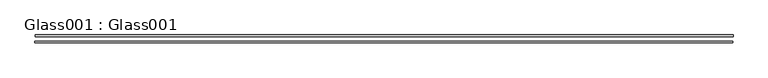
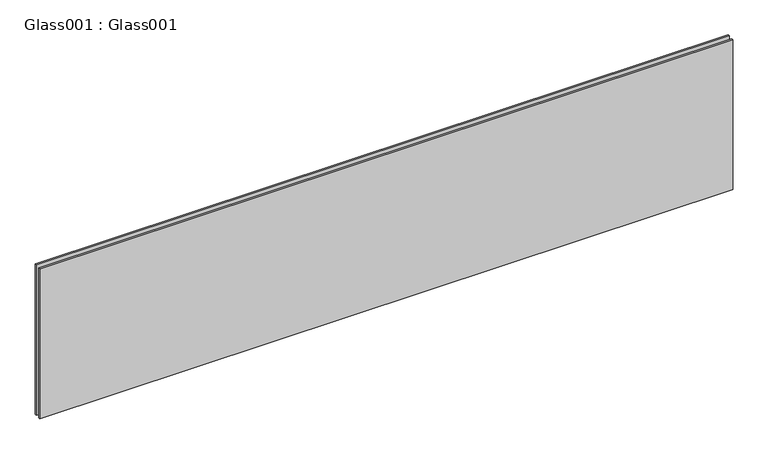
"""IFC4 building model written with IfcOpenShell, lengths in millimetres: proxy geometry, Glass001 : Glass001."""

import ifcopenshell
import ifcopenshell.guid

model = None  # the IFC model being written
_history = None  # IfcOwnerHistory: only IFC2X3 demands one
_inside = {}  # id of a spatial element -> (the spatial element, [elements in it])
_under = {}  # id of a project, library or spatial element -> (it, [spatial elements below it])
_declared = {}  # id of a project -> (the project, [libraries it declares])
_typed = {}  # id of a type object -> (the type object, [elements of that type])
_made_of = {}  # id of a material, layer set ... -> (it, [elements and type objects made of it])


def new_model(schema):
    """Start an empty IFC model of exactly this schema.

    Asked for "IFC4X3", IfcOpenShell would pick the latest addendum, in which some entities
    have other attributes; the version numbers below select the first issue.
    IFC2X3 requires an IfcOwnerHistory on every rooted entity: one is made here for all.
    """
    global model, _history
    if schema == "IFC4X3":
        model = ifcopenshell.file(schema_version=(4, 3, 0, 0))
    else:
        model = ifcopenshell.file(schema=schema)
    _inside.clear()
    _under.clear()
    _declared.clear()
    _typed.clear()
    _made_of.clear()
    _history = None
    if model.schema == "IFC2X3":
        org = make("IfcOrganization", Name="unknown")
        user = make(
            "IfcPersonAndOrganization",
            ThePerson=make("IfcPerson", FamilyName="unknown"),
            TheOrganization=org,
        )
        app = make(
            "IfcApplication",
            ApplicationDeveloper=org,
            Version="unknown",
            ApplicationFullName="unknown",
            ApplicationIdentifier="unknown",
        )
        _history = make(
            "IfcOwnerHistory",
            OwningUser=user,
            OwningApplication=app,
            ChangeAction="ADDED",
            CreationDate=0,
        )
    return model


def make(cls, **values):
    """One entity of the class cls with the attributes given. An attribute that is None is left unset."""
    return model.create_entity(
        cls, **{name: value for name, value in values.items() if value is not None}
    )


def rooted(cls, **values):
    """An entity with a GlobalId (a new one), such as an element, a storey or a relation."""
    return make(cls, GlobalId=ifcopenshell.guid.new(), OwnerHistory=_history, **values)


def si_unit(unit_type, name, prefix=None):
    """IfcSIUnit, for example si_unit("LENGTHUNIT", "METRE", prefix="MILLI")."""
    return make("IfcSIUnit", UnitType=unit_type, Prefix=prefix, Name=name)


def assignment(units):
    """IfcUnitAssignment: the units of a project."""
    return None if units is None else make("IfcUnitAssignment", Units=units)


def point(xyz):
    """IfcCartesianPoint."""
    return None if xyz is None else make("IfcCartesianPoint", Coordinates=xyz)


def direction(xyz):
    """IfcDirection."""
    return None if xyz is None else make("IfcDirection", DirectionRatios=xyz)


def frame(location, z_axis=None, x_axis=None):
    """IfcAxis2Placement3D, a coordinate frame: its origin and axes. An axis left out is left unset."""
    return make(
        "IfcAxis2Placement3D",
        Location=point(location),
        Axis=direction(z_axis),
        RefDirection=direction(x_axis),
    )


def origin():
    """The frame at (0, 0, 0) with its axes left unset."""
    return frame((0.0, 0.0, 0.0))


def place(relative_to, where):
    """IfcLocalPlacement: puts the frame where relative to a parent placement (None: the world)."""
    return make(
        "IfcLocalPlacement", PlacementRelTo=relative_to, RelativePlacement=where
    )


def context(
    kind, dimensions, precision=None, world=None, true_north=None, identifier=None
):
    """IfcGeometricRepresentationContext, for example the 3D "Model" context."""
    return make(
        "IfcGeometricRepresentationContext",
        ContextIdentifier=identifier,
        ContextType=kind,
        CoordinateSpaceDimension=dimensions,
        Precision=precision,
        WorldCoordinateSystem=world,
        TrueNorth=true_north,
    )


def project(units=None, contexts=None):
    """IfcProject with its units and contexts."""
    return rooted(
        "IfcProject",
        Name="project",
        RepresentationContexts=contexts,
        UnitsInContext=assignment(units),
    )


def spatial(cls, under=None, at=None, **own):
    """A site, building, storey or space (cls), placed at a placement, below another one or the project."""
    s = rooted(cls, ObjectPlacement=at, **own)
    if under is not None:
        _under.setdefault(under.id(), (under, []))[1].append(s)
    return s


def polyline(points):
    """IfcPolyline through the points."""
    return make("IfcPolyline", Points=[point(p) for p in points])


def outline(outer, holes=None, kind="AREA"):
    """IfcArbitraryClosedProfileDef: a profile drawn as a closed curve; with holes, ...WithVoids."""
    if holes is None:
        return make("IfcArbitraryClosedProfileDef", ProfileType=kind, OuterCurve=outer)
    return make(
        "IfcArbitraryProfileDefWithVoids",
        ProfileType=kind,
        OuterCurve=outer,
        InnerCurves=holes,
    )


def extrude(swept, where, along, depth):
    """IfcExtrudedAreaSolid: the profile swept, set in the frame where, extruded along a direction by depth."""
    return make(
        "IfcExtrudedAreaSolid",
        SweptArea=swept,
        Position=where,
        ExtrudedDirection=direction(along),
        Depth=depth,
    )


def shape(context_of_items, identifier, shape_type, items):
    """IfcShapeRepresentation: the items that make up one representation, for example the "Body"."""
    return make(
        "IfcShapeRepresentation",
        ContextOfItems=context_of_items,
        RepresentationIdentifier=identifier,
        RepresentationType=shape_type,
        Items=items,
    )


def source(mapping_origin, context_of_items, identifier, shape_type, items):
    """IfcRepresentationMap: a shape defined once, which mapped items show again and again."""
    return make(
        "IfcRepresentationMap",
        MappingOrigin=mapping_origin,
        MappedRepresentation=shape(context_of_items, identifier, shape_type, items),
    )


def transform(
    local_origin,
    x_axis=None,
    y_axis=None,
    z_axis=None,
    scale=None,
    scale2=None,
    scale3=None,
    uniform=True,
):
    """IfcCartesianTransformationOperator3D, or its non-uniform kind. x_axis, y_axis, z_axis: its Axis1, 2, 3."""
    if uniform:
        return make(
            "IfcCartesianTransformationOperator3D",
            Axis1=direction(x_axis),
            Axis2=direction(y_axis),
            LocalOrigin=point(local_origin),
            Scale=scale,
            Axis3=direction(z_axis),
        )
    return make(
        "IfcCartesianTransformationOperator3DnonUniform",
        Axis1=direction(x_axis),
        Axis2=direction(y_axis),
        LocalOrigin=point(local_origin),
        Scale=scale,
        Axis3=direction(z_axis),
        Scale2=scale2,
        Scale3=scale3,
    )


def mapped(mapping_source, mapping_target):
    """IfcMappedItem: shows the shape of a source again, moved by a transform."""
    return make(
        "IfcMappedItem", MappingSource=mapping_source, MappingTarget=mapping_target
    )


def made_of(thing, what):
    """Note that an element or type object is made of a material, layer set ...; save() writes the relation."""
    if what is not None:
        _made_of.setdefault(what.id(), (what, []))[1].append(thing)
    return thing


def element(
    cls,
    number,
    at=None,
    inside=None,
    cuts=None,
    type_object=None,
    material=None,
    context=None,
    identifier="Body",
    shape_type=None,
    held_by="IfcProductDefinitionShape",
    body=None,
    shapes=None,
    **own,
):
    """One element of the class cls, such as IfcWall. Its Tag is "e" and its number.

    at: its placement. inside: the storey or other place that contains it. cuts: it is an
    opening in that element (IfcRelVoidsElement). A single representation is given by context,
    identifier, shape_type and body (its items); several are given by shapes. held_by: the class
    of the entity that holds the representations. save() writes the other relations.
    """
    e = rooted(cls, Tag="e%d" % number, ObjectPlacement=at, **own)
    if body is not None:
        shapes = [shape(context, identifier, shape_type, body)]
    if shapes is not None:
        e.Representation = make(held_by, Representations=shapes)
    if inside is not None:
        _inside.setdefault(inside.id(), (inside, []))[1].append(e)
    if cuts is not None:
        rooted(
            "IfcRelVoidsElement", RelatingBuildingElement=cuts, RelatedOpeningElement=e
        )
    if type_object is not None:
        _typed.setdefault(type_object.id(), (type_object, []))[1].append(e)
    return made_of(e, material)


def aggregate(whole, parts):
    """IfcRelAggregates: a whole, such as a stair, and the parts it consists of."""
    return rooted("IfcRelAggregates", RelatingObject=whole, RelatedObjects=parts)


def save(model, path):
    """Write the relations noted so far, then the file.

    IfcRelAggregates (storeys below a building ...), IfcRelContainedInSpatialStructure (elements
    in a storey), IfcRelDefinesByType, IfcRelAssociatesMaterial and IfcRelDeclares: one each for
    every whole, place, type object, material and project.
    """
    for whole, parts in _under.values():
        aggregate(whole, parts)
    for where, things in _inside.values():
        rooted(
            "IfcRelContainedInSpatialStructure",
            RelatedElements=things,
            RelatingStructure=where,
        )
    for kind, things in _typed.values():
        rooted("IfcRelDefinesByType", RelatedObjects=things, RelatingType=kind)
    for what, things in _made_of.values():
        rooted("IfcRelAssociatesMaterial", RelatedObjects=things, RelatingMaterial=what)
    for by, libraries in _declared.values():
        rooted("IfcRelDeclares", RelatingContext=by, RelatedDefinitions=libraries)
    model.write(path)


def glass001_glass001_dcca6a89(model_context):
    return source(origin(), model_context, "Body", "SweptSolid", [
        extrude(outline(polyline([(14384.0178845, -4642.8027938), (14384.0178845, -4647.8027938), (12384.0178845, -4647.8027938), (12384.0178845, -4642.8027938), (14384.0178845, -4642.8027938)])), frame((0.0, 0.0, 38486.2565625), z_axis=(0.0, 0.0, 1.0), x_axis=(1.0, 0.0, 0.0)), (0.0, 0.0, 1.0), 457.9389687),
        extrude(outline(polyline([(14383.0178845, -4660.8027938), (14383.0178845, -4665.8027938), (12383.0178845, -4665.8027938), (12383.0178845, -4660.8027938), (14383.0178845, -4660.8027938)])), frame((0.0, 0.0, 38486.2565625), z_axis=(0.0, 0.0, 1.0), x_axis=(1.0, 0.0, 0.0)), (0.0, 0.0, 1.0), 457.9389687),
    ])


if __name__ == "__main__":
    model = new_model("IFC4")
    model_context = context("Model", 3, world=origin())
    ifc_project = project(units=[si_unit("LENGTHUNIT", "METRE", prefix="MILLI")], contexts=[model_context])
    site = spatial("IfcSite", under=ifc_project)
    building = spatial("IfcBuilding", under=site)
    placement = place(None, origin())
    glass001_glass001_shape = glass001_glass001_dcca6a89(model_context)
    element("IfcBuildingElementProxy", 1, Name="Glass001 : Glass001", ObjectType="Glass001 : Glass001", at=placement, inside=building, context=model_context, shape_type="MappedRepresentation", body=[
        mapped(glass001_glass001_shape, transform((0.0, 0.0, 0.0), x_axis=(1.0, 0.0, 0.0), y_axis=(0.0, 1.0, 0.0), z_axis=(0.0, 0.0, 1.0))),
    ])
    save(model, "model.ifc")

# Revit data of these elements
# Type "Glass001 : Glass001"
#   NameOverride = "Glass001"
# Element 1 (IfcBuildingElementProxy, "Glass001 : Glass001")
#   Materials on its faces: "1\"  INSULATED GLAZING"
# Materials
#   "1\"  INSULATED GLAZING": class "Unassigned", colour RGB 146 199 212, transparency 0, Cost = 0
